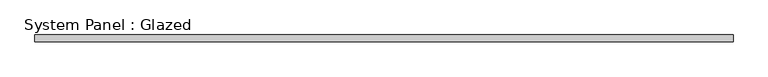
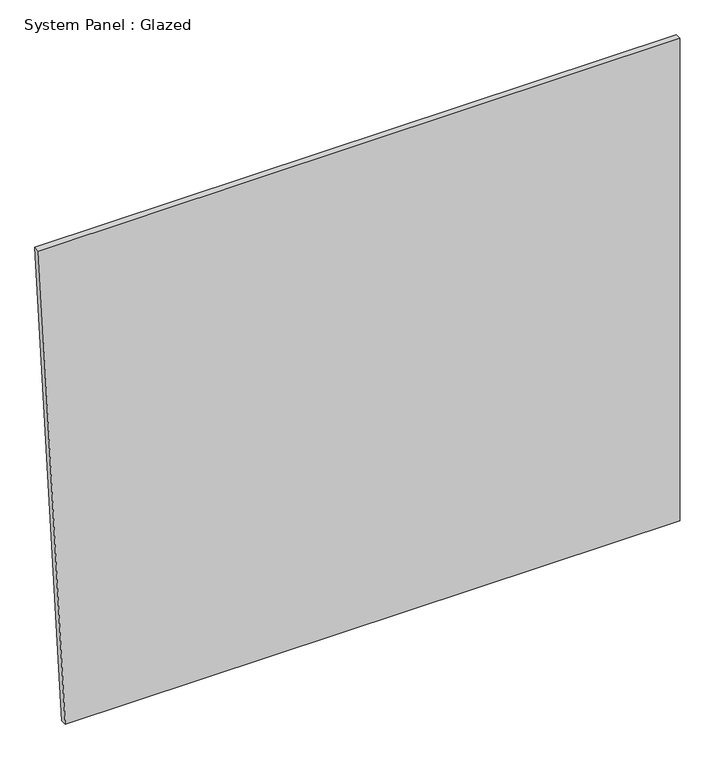
"""IFC4 building model written with IfcOpenShell, lengths in millimetres: plate geometry, System Panel : Glazed."""

import ifcopenshell
import ifcopenshell.guid

model = None  # the IFC model being written
_history = None  # IfcOwnerHistory: only IFC2X3 demands one
_inside = {}  # id of a spatial element -> (the spatial element, [elements in it])
_under = {}  # id of a project, library or spatial element -> (it, [spatial elements below it])
_declared = {}  # id of a project -> (the project, [libraries it declares])
_typed = {}  # id of a type object -> (the type object, [elements of that type])
_made_of = {}  # id of a material, layer set ... -> (it, [elements and type objects made of it])


def new_model(schema):
    """Start an empty IFC model of exactly this schema.

    Asked for "IFC4X3", IfcOpenShell would pick the latest addendum, in which some entities
    have other attributes; the version numbers below select the first issue.
    IFC2X3 requires an IfcOwnerHistory on every rooted entity: one is made here for all.
    """
    global model, _history
    if schema == "IFC4X3":
        model = ifcopenshell.file(schema_version=(4, 3, 0, 0))
    else:
        model = ifcopenshell.file(schema=schema)
    _inside.clear()
    _under.clear()
    _declared.clear()
    _typed.clear()
    _made_of.clear()
    _history = None
    if model.schema == "IFC2X3":
        org = make("IfcOrganization", Name="unknown")
        user = make(
            "IfcPersonAndOrganization",
            ThePerson=make("IfcPerson", FamilyName="unknown"),
            TheOrganization=org,
        )
        app = make(
            "IfcApplication",
            ApplicationDeveloper=org,
            Version="unknown",
            ApplicationFullName="unknown",
            ApplicationIdentifier="unknown",
        )
        _history = make(
            "IfcOwnerHistory",
            OwningUser=user,
            OwningApplication=app,
            ChangeAction="ADDED",
            CreationDate=0,
        )
    return model


def make(cls, **values):
    """One entity of the class cls with the attributes given. An attribute that is None is left unset."""
    return model.create_entity(
        cls, **{name: value for name, value in values.items() if value is not None}
    )


def rooted(cls, **values):
    """An entity with a GlobalId (a new one), such as an element, a storey or a relation."""
    return make(cls, GlobalId=ifcopenshell.guid.new(), OwnerHistory=_history, **values)


def si_unit(unit_type, name, prefix=None):
    """IfcSIUnit, for example si_unit("LENGTHUNIT", "METRE", prefix="MILLI")."""
    return make("IfcSIUnit", UnitType=unit_type, Prefix=prefix, Name=name)


def assignment(units):
    """IfcUnitAssignment: the units of a project."""
    return None if units is None else make("IfcUnitAssignment", Units=units)


def point(xyz):
    """IfcCartesianPoint."""
    return None if xyz is None else make("IfcCartesianPoint", Coordinates=xyz)


def direction(xyz):
    """IfcDirection."""
    return None if xyz is None else make("IfcDirection", DirectionRatios=xyz)


def frame(location, z_axis=None, x_axis=None):
    """IfcAxis2Placement3D, a coordinate frame: its origin and axes. An axis left out is left unset."""
    return make(
        "IfcAxis2Placement3D",
        Location=point(location),
        Axis=direction(z_axis),
        RefDirection=direction(x_axis),
    )


def origin():
    """The frame at (0, 0, 0) with its axes left unset."""
    return frame((0.0, 0.0, 0.0))


def place(relative_to, where):
    """IfcLocalPlacement: puts the frame where relative to a parent placement (None: the world)."""
    return make(
        "IfcLocalPlacement", PlacementRelTo=relative_to, RelativePlacement=where
    )


def context(
    kind, dimensions, precision=None, world=None, true_north=None, identifier=None
):
    """IfcGeometricRepresentationContext, for example the 3D "Model" context."""
    return make(
        "IfcGeometricRepresentationContext",
        ContextIdentifier=identifier,
        ContextType=kind,
        CoordinateSpaceDimension=dimensions,
        Precision=precision,
        WorldCoordinateSystem=world,
        TrueNorth=true_north,
    )


def project(units=None, contexts=None):
    """IfcProject with its units and contexts."""
    return rooted(
        "IfcProject",
        Name="project",
        RepresentationContexts=contexts,
        UnitsInContext=assignment(units),
    )


def spatial(cls, under=None, at=None, **own):
    """A site, building, storey or space (cls), placed at a placement, below another one or the project."""
    s = rooted(cls, ObjectPlacement=at, **own)
    if under is not None:
        _under.setdefault(under.id(), (under, []))[1].append(s)
    return s


def polyline(points):
    """IfcPolyline through the points."""
    return make("IfcPolyline", Points=[point(p) for p in points])


def outline(outer, holes=None, kind="AREA"):
    """IfcArbitraryClosedProfileDef: a profile drawn as a closed curve; with holes, ...WithVoids."""
    if holes is None:
        return make("IfcArbitraryClosedProfileDef", ProfileType=kind, OuterCurve=outer)
    return make(
        "IfcArbitraryProfileDefWithVoids",
        ProfileType=kind,
        OuterCurve=outer,
        InnerCurves=holes,
    )


def extrude(swept, where, along, depth):
    """IfcExtrudedAreaSolid: the profile swept, set in the frame where, extruded along a direction by depth."""
    return make(
        "IfcExtrudedAreaSolid",
        SweptArea=swept,
        Position=where,
        ExtrudedDirection=direction(along),
        Depth=depth,
    )


def shape(context_of_items, identifier, shape_type, items):
    """IfcShapeRepresentation: the items that make up one representation, for example the "Body"."""
    return make(
        "IfcShapeRepresentation",
        ContextOfItems=context_of_items,
        RepresentationIdentifier=identifier,
        RepresentationType=shape_type,
        Items=items,
    )


def source(mapping_origin, context_of_items, identifier, shape_type, items):
    """IfcRepresentationMap: a shape defined once, which mapped items show again and again."""
    return make(
        "IfcRepresentationMap",
        MappingOrigin=mapping_origin,
        MappedRepresentation=shape(context_of_items, identifier, shape_type, items),
    )


def transform(
    local_origin,
    x_axis=None,
    y_axis=None,
    z_axis=None,
    scale=None,
    scale2=None,
    scale3=None,
    uniform=True,
):
    """IfcCartesianTransformationOperator3D, or its non-uniform kind. x_axis, y_axis, z_axis: its Axis1, 2, 3."""
    if uniform:
        return make(
            "IfcCartesianTransformationOperator3D",
            Axis1=direction(x_axis),
            Axis2=direction(y_axis),
            LocalOrigin=point(local_origin),
            Scale=scale,
            Axis3=direction(z_axis),
        )
    return make(
        "IfcCartesianTransformationOperator3DnonUniform",
        Axis1=direction(x_axis),
        Axis2=direction(y_axis),
        LocalOrigin=point(local_origin),
        Scale=scale,
        Axis3=direction(z_axis),
        Scale2=scale2,
        Scale3=scale3,
    )


def mapped(mapping_source, mapping_target):
    """IfcMappedItem: shows the shape of a source again, moved by a transform."""
    return make(
        "IfcMappedItem", MappingSource=mapping_source, MappingTarget=mapping_target
    )


def made_of(thing, what):
    """Note that an element or type object is made of a material, layer set ...; save() writes the relation."""
    if what is not None:
        _made_of.setdefault(what.id(), (what, []))[1].append(thing)
    return thing


def element(
    cls,
    number,
    at=None,
    inside=None,
    cuts=None,
    type_object=None,
    material=None,
    context=None,
    identifier="Body",
    shape_type=None,
    held_by="IfcProductDefinitionShape",
    body=None,
    shapes=None,
    **own,
):
    """One element of the class cls, such as IfcWall. Its Tag is "e" and its number.

    at: its placement. inside: the storey or other place that contains it. cuts: it is an
    opening in that element (IfcRelVoidsElement). A single representation is given by context,
    identifier, shape_type and body (its items); several are given by shapes. held_by: the class
    of the entity that holds the representations. save() writes the other relations.
    """
    e = rooted(cls, Tag="e%d" % number, ObjectPlacement=at, **own)
    if body is not None:
        shapes = [shape(context, identifier, shape_type, body)]
    if shapes is not None:
        e.Representation = make(held_by, Representations=shapes)
    if inside is not None:
        _inside.setdefault(inside.id(), (inside, []))[1].append(e)
    if cuts is not None:
        rooted(
            "IfcRelVoidsElement", RelatingBuildingElement=cuts, RelatedOpeningElement=e
        )
    if type_object is not None:
        _typed.setdefault(type_object.id(), (type_object, []))[1].append(e)
    return made_of(e, material)


def aggregate(whole, parts):
    """IfcRelAggregates: a whole, such as a stair, and the parts it consists of."""
    return rooted("IfcRelAggregates", RelatingObject=whole, RelatedObjects=parts)


def save(model, path):
    """Write the relations noted so far, then the file.

    IfcRelAggregates (storeys below a building ...), IfcRelContainedInSpatialStructure (elements
    in a storey), IfcRelDefinesByType, IfcRelAssociatesMaterial and IfcRelDeclares: one each for
    every whole, place, type object, material and project.
    """
    for whole, parts in _under.values():
        aggregate(whole, parts)
    for where, things in _inside.values():
        rooted(
            "IfcRelContainedInSpatialStructure",
            RelatedElements=things,
            RelatingStructure=where,
        )
    for kind, things in _typed.values():
        rooted("IfcRelDefinesByType", RelatedObjects=things, RelatingType=kind)
    for what, things in _made_of.values():
        rooted("IfcRelAssociatesMaterial", RelatedObjects=things, RelatingMaterial=what)
    for by, libraries in _declared.values():
        rooted("IfcRelDeclares", RelatingContext=by, RelatedDefinitions=libraries)
    model.write(path)


def system_panel_glazed_02f5044a(model_context):
    return source(origin(), model_context, "Body", "SweptSolid", [
        extrude(outline(polyline([(0.0, -1204.0949696), (0.0, 1313.2352527), (2085.3785982, 1313.2352527), (2085.3785982, -1313.2352527), (0.0, -1204.0949696)])), frame((0.0, -44.45, 0.0), z_axis=(0.0, 1.0, 0.0), x_axis=(0.0, 0.0, 1.0)), (0.0, 0.0, 1.0), 25.4),
    ])


if __name__ == "__main__":
    model = new_model("IFC4")
    model_context = context("Model", 3, world=origin())
    ifc_project = project(units=[si_unit("LENGTHUNIT", "METRE", prefix="MILLI")], contexts=[model_context])
    site = spatial("IfcSite", under=ifc_project)
    building = spatial("IfcBuilding", under=site)
    placement = place(None, origin())
    system_panel_glazed_shape = system_panel_glazed_02f5044a(model_context)
    element("IfcPlate", 1, ObjectType="System Panel : Glazed", at=placement, inside=building, context=model_context, shape_type="MappedRepresentation", body=[
        mapped(system_panel_glazed_shape, transform((0.0, 0.0, 0.0), x_axis=(1.0, 0.0, 0.0), y_axis=(0.0, 1.0, 0.0), z_axis=(0.0, 0.0, 1.0))),
    ])
    save(model, "model.ifc")

# Revit data of these elements
# Project information
#   Organization Name = "G3B Press"
#   Organization Description = "Paul F. Aubin Cosulting Services, Inc."
#   Building Name = "Revit Essentials for Architecture"
#   Author = "Paul F. Aubin"
#   Author Website = "https://www.paulaubin.com"
#   Copyright = "Copyright © 2020 Paul F Aubin, all rights reserved"
#   Design Option = "Main Model"
#   Project Issue Date = "8/1/2020"
#   Project Status = "Design Development"
#   Client Name = "Rendering and Presentation"
#   Project Address = "123 State ST\nSuite 301\nChicago, IL 60606"
#   Project Name = "18 Commercial"
#   Project Number = "2020.04A"
# Type "System Panel : Glazed"
#   Construction Type Id = "GSP4R"
#   Analytic Construction = "1/8 in Pilkington single glazing"
#   Visual Light Transmittance = 0.9
#   Solar Heat Gain Coefficient = 0.86
#   Heat Transfer Coefficient (U) = 1.18115 BTU/(h·ft²·°F)
#   Define Thermal Properties by = 1
# Element 1 (IfcPlate, "System Panel : Glazed")
#   Materials on its faces: "Glass"
# Materials
#   "Glass": class "Glass", colour RGB 0 128 192, transparency 0.75, Description = "Soda Lime Glass", Cost = 0
